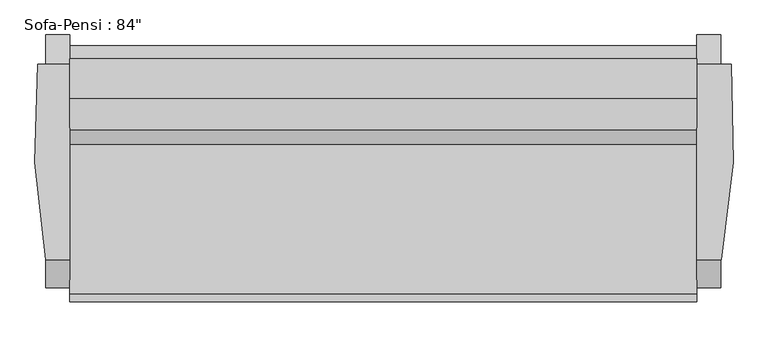
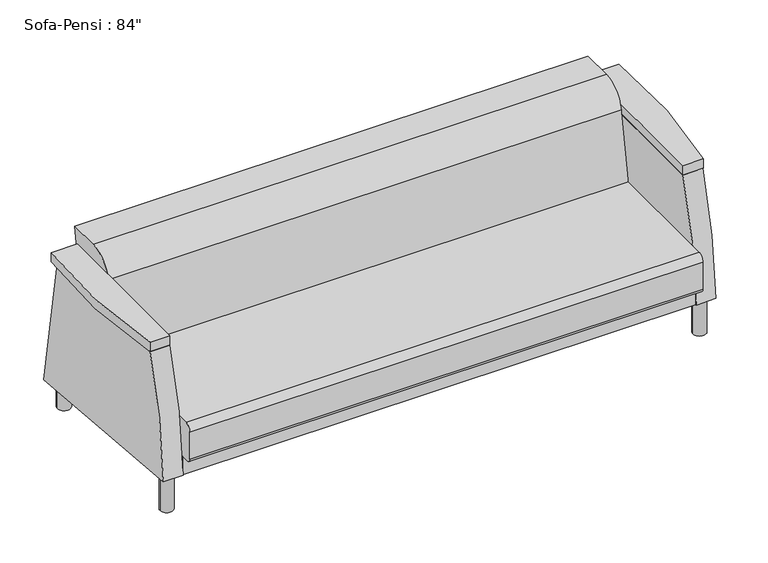
"""IFC4 building model written with IfcOpenShell, lengths in millimetres: furniture geometry."""

from ifc_helpers import new_model, si_unit, point, frame, frame_2d, origin, origin_with_axes, place, context, project, spatial, polyline, circle_curve, trimmed, segment, composite_curve, outline, extrude, source, transform, mapped, element, save


def furniture_fb1f61f5(model_context):
    return source(origin(), model_context, "Body", "SweptSolid", [
        extrude(outline(composite_curve([segment(trimmed(circle_curve(frame_2d((-750.09375, -53.0901639)), 25.4), [point((-775.49375, -53.0901639))], [point((-724.69375, -53.0901639))], False, "CARTESIAN"), True, "CONTINUOUS"), segment(trimmed(circle_curve(frame_2d((-750.09375, -53.0901639)), 25.4), [point((-724.69375, -53.0901639))], [point((-775.49375, -53.0901639))], False, "CARTESIAN"), True, "CONTINUOUS")], self_intersect=False)), origin_with_axes(), (0.0, 0.0, 1.0), 148.43125),
        extrude(outline(composite_curve([segment(trimmed(circle_curve(frame_2d((-750.09375, 632.7098361)), 25.4), [point((-775.49375, 632.7098361))], [point((-724.69375, 632.7098361))], False, "CARTESIAN"), True, "CONTINUOUS"), segment(trimmed(circle_curve(frame_2d((-750.09375, 632.7098361)), 25.4), [point((-724.69375, 632.7098361))], [point((-775.49375, 632.7098361))], False, "CARTESIAN"), True, "CONTINUOUS")], self_intersect=False)), origin_with_axes(), (0.0, 0.0, 1.0), 148.43125),
        extrude(outline(composite_curve([segment(trimmed(circle_curve(frame_2d((1307.30625, 632.7098361)), 25.4), [point((1281.90625, 632.7098361))], [point((1332.70625, 632.7098361))], False, "CARTESIAN"), True, "CONTINUOUS"), segment(trimmed(circle_curve(frame_2d((1307.30625, 632.7098361)), 25.4), [point((1332.70625, 632.7098361))], [point((1281.90625, 632.7098361))], False, "CARTESIAN"), True, "CONTINUOUS")], self_intersect=False)), origin_with_axes(), (0.0, 0.0, 1.0), 148.43125),
        extrude(outline(composite_curve([segment(trimmed(circle_curve(frame_2d((1307.30625, -53.0901639)), 25.4), [point((1281.90625, -53.0901639))], [point((1332.70625, -53.0901639))], False, "CARTESIAN"), True, "CONTINUOUS"), segment(trimmed(circle_curve(frame_2d((1307.30625, -53.0901639)), 25.4), [point((1332.70625, -53.0901639))], [point((1281.90625, -53.0901639))], False, "CARTESIAN"), True, "CONTINUOUS")], self_intersect=False)), origin_with_axes(), (0.0, 0.0, 1.0), 148.43125),
        extrude(outline(polyline([(1269.20625, 668.3047863), (1269.20625, -93.6952137), (-711.99375, -93.6952137), (-711.99375, 668.3047863), (1269.20625, 668.3047863)])), frame((0.0, 0.0, 148.0509954), z_axis=(0.0, 0.0, 1.0), x_axis=(1.0, 0.0, 0.0)), (0.0, 0.0, 1.0), 76.2),
        extrude(outline(composite_curve([segment(polyline([(-9.3943348, 626.0203985), (608.6917937, 626.0203985), (701.7619204, 79.3588346), (-97.7900405, 149.3105671)]), True, "CONTINUOUS"), segment(trimmed(circle_curve(frame_2d((1499.9783711, 99.5888442)), 1598.5418814), [point((-97.7900405, 149.3105671))], [point((-9.3943348, 626.0203985))], False, "CARTESIAN"), True, "CONTINUOUS")], self_intersect=False)), frame((-788.19375, 0.0, 0.0), z_axis=(1.0, 0.0, 0.0), x_axis=(0.0, 1.0, 0.0)), (0.0, 0.0, 1.0), 76.2),
        extrude(outline(composite_curve([segment(polyline([(701.7619204, 79.3588346), (-97.7900405, 149.3105671)]), True, "CONTINUOUS"), segment(trimmed(circle_curve(frame_2d((1499.9783711, 99.5888442)), 1598.5418814), [point((-97.7900405, 149.3105671))], [point((-9.3943348, 626.0203985))], False, "CARTESIAN"), True, "CONTINUOUS"), segment(polyline([(-9.3943348, 626.0203985), (608.6917937, 626.0203985), (701.7619204, 79.3588346)]), True, "CONTINUOUS")], self_intersect=False)), frame((1269.20625, 0.0, 0.0), z_axis=(1.0, 0.0, 0.0), x_axis=(0.0, 1.0, 0.0)), (0.0, 0.0, 1.0), 76.2),
        extrude(outline(composite_curve([segment(trimmed(circle_curve(frame_2d((-116.5901639, 351.2509954)), 25.4), [point((-141.9901639, 351.2509954))], [point((-116.5901639, 376.6509954))], False, "CARTESIAN"), True, "CONTINUOUS"), segment(polyline([(-116.5901639, 376.6509954), (355.3895541, 376.6509954), (402.1988177, 642.1195211)]), True, "CONTINUOUS"), segment(trimmed(circle_curve(frame_2d((502.2552854, 624.4768662)), 101.6), [point((402.1988177, 642.1195211))], [point((502.2552854, 726.0768662))], False, "CARTESIAN"), True, "CONTINUOUS"), segment(polyline([(502.2552854, 726.0768662), (626.3344485, 726.0768662), (609.5377828, 620.1719187), (667.6541767, 224.2509954), (-126.1151639, 224.2509954)]), True, "CONTINUOUS"), segment(trimmed(circle_curve(frame_2d((-126.1151639, 240.1259954)), 15.875), [point((-126.1151639, 224.2509954))], [point((-141.9901639, 240.1259954))], False, "CARTESIAN"), True, "CONTINUOUS"), segment(polyline([(-141.9901639, 240.1259954), (-141.9901639, 351.2509954)]), True, "CONTINUOUS")], self_intersect=False)), frame((-711.99375, 0.0, 0.0), z_axis=(1.0, 0.0, 0.0), x_axis=(0.0, 1.0, 0.0)), (0.0, 0.0, 1.0), 1981.2),
        extrude(outline(composite_curve([segment(polyline([(-711.99375, -9.3943348), (-788.19375, -9.3943348)]), True, "CONTINUOUS"), segment(trimmed(circle_curve(frame_2d((1379.5527561, 389.2532985)), 2204.0972869), [point((-788.19375, -9.3943348))], [point((-813.59375, 608.6917935))], False, "CARTESIAN"), True, "CONTINUOUS"), segment(polyline([(-813.59375, 608.6917935), (-711.99375, 608.6917935), (-711.99375, -9.3943348)]), True, "CONTINUOUS")], self_intersect=False)), frame((0.0, 0.0, 626.0203985), z_axis=(0.0, 0.0, 1.0), x_axis=(1.0, 0.0, 0.0)), (0.0, 0.0, 1.0), 38.1),
        extrude(outline(composite_curve([segment(polyline([(1269.20625, -9.3943348), (1269.20625, 608.9395268), (1377.8864453, 608.9395268)]), True, "CONTINUOUS"), segment(trimmed(circle_curve(frame_2d((-821.3771494, 407.0073811)), 2208.514648), [point((1377.8864453, 608.9395268))], [point((1347.5273117, -9.3943348))], False, "CARTESIAN"), True, "CONTINUOUS"), segment(polyline([(1347.5273117, -9.3943348), (1269.20625, -9.3943348)]), True, "CONTINUOUS")], self_intersect=False)), frame((0.0, 0.0, 626.0203985), z_axis=(0.0, 0.0, 1.0), x_axis=(1.0, 0.0, 0.0)), (0.0, 0.0, 1.0), 38.1),
    ])


if __name__ == "__main__":
    model = new_model("IFC4")
    model_context = context("Model", 3, world=origin())
    ifc_project = project(units=[si_unit("LENGTHUNIT", "METRE", prefix="MILLI")], contexts=[model_context])
    site = spatial("IfcSite", under=ifc_project)
    building = spatial("IfcBuilding", under=site)
    placement = place(None, origin())
    furniture_shape = furniture_fb1f61f5(model_context)
    element("IfcFurniture", 1, ObjectType="Sofa-Pensi : 84\"", at=placement, inside=building, context=model_context, shape_type="MappedRepresentation", body=[
        mapped(furniture_shape, transform((0.0, 0.0, 0.0), x_axis=(1.0, 0.0, 0.0), y_axis=(0.0, 1.0, 0.0), z_axis=(0.0, 0.0, 1.0))),
    ])
    save(model, "model.ifc")

# Revit data of these elements
# Type "Sofa-Pensi : 84\""
#   Assembly Code = "E2020200"
#   Length = 7' - 0"
#   Frame Material = Wood - Cherry
#   Seat Material = Textile - Linen, Smooth
#   Feet Material = Metal - Chrome
# Element 1 (IfcFurniture, "Sofa-Pensi : 84\"")
#   Materials on its faces: "Wood - Cherry", "Textile - Linen, Smooth", "Metal - Chrome"
# Materials
#   "Wood - Cherry": class "Wood", colour RGB 192 120 57, transparency 0, Comments = "Rendering appearance not upgraded Rendering appearance not upgraded ", Description = "Cherry"
#   "Textile - Linen, Smooth": class "Fabric", colour RGB 189 191 172, transparency 0, Comments = "Rendering appearance not upgraded Rendering appearance not upgraded "
#   "Metal - Chrome": class "Metal", colour RGB 244 244 244, transparency 0, Comments = "Rendering appearance not upgraded Rendering appearance not upgraded ", Description = "Chrome"
